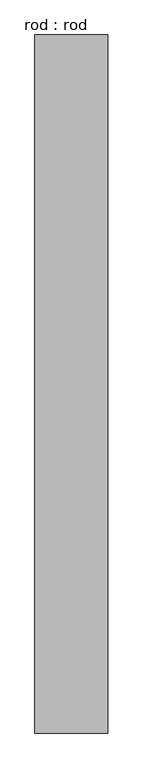
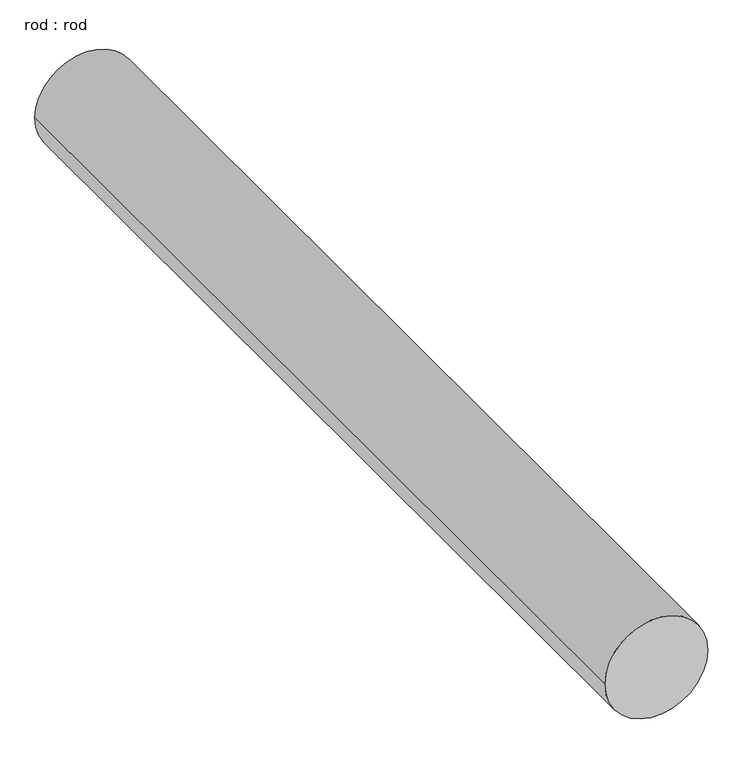
"""IFC4 building model written with IfcOpenShell, lengths in millimetres: proxy geometry, rod : rod."""

from ifc_helpers import new_model, si_unit, point, frame, frame_2d, origin, place, context, project, spatial, circle_curve, trimmed, segment, composite_curve, outline, extrude, source, transform, mapped, element, save


def rod_rod_0e2c7b4d(model_context):
    return source(origin(), model_context, "Body", "SweptSolid", [
        extrude(outline(composite_curve([segment(trimmed(circle_curve(frame_2d((0.0108462, 0.0)), 200.0), [point((0.0108462, 200.0))], [point((0.0108462, -200.0))], False, "CARTESIAN"), True, "CONTINUOUS"), segment(trimmed(circle_curve(frame_2d((0.0108462, 0.0)), 200.0), [point((0.0108462, -200.0))], [point((0.0108462, 200.0))], False, "CARTESIAN"), True, "CONTINUOUS")], self_intersect=False)), frame((0.0, 2178.2688351, 0.0), z_axis=(0.0, 1.0, 0.0), x_axis=(0.0, 0.0, 1.0)), (0.0, 0.0, 1.0), 3828.9195604),
    ])


if __name__ == "__main__":
    model = new_model("IFC4")
    model_context = context("Model", 3, world=origin())
    ifc_project = project(units=[si_unit("LENGTHUNIT", "METRE", prefix="MILLI")], contexts=[model_context])
    site = spatial("IfcSite", under=ifc_project)
    building = spatial("IfcBuilding", under=site)
    placement = place(None, origin())
    rod_rod_shape = rod_rod_0e2c7b4d(model_context)
    element("IfcBuildingElementProxy", 1, Name="rod : rod", ObjectType="rod : rod", at=placement, inside=building, context=model_context, shape_type="MappedRepresentation", body=[
        mapped(rod_rod_shape, transform((0.0, 0.0, 0.0), x_axis=(1.0, 0.0, 0.0), y_axis=(0.0, 1.0, 0.0), z_axis=(0.0, 0.0, 1.0))),
    ])
    save(model, "model.ifc")

# Revit data of these elements
# Type "rod : rod"
#   Default Elevation = 0
